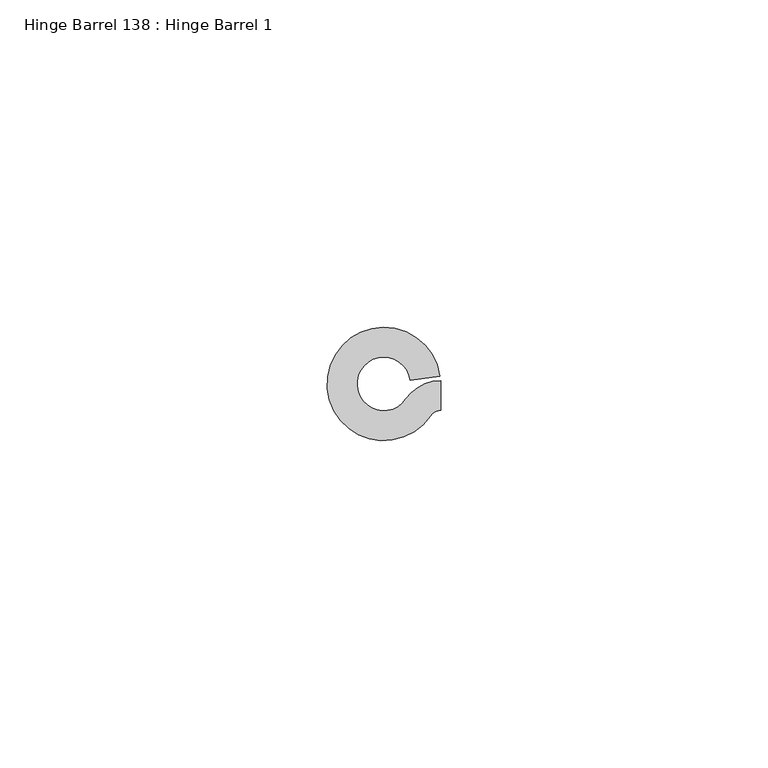
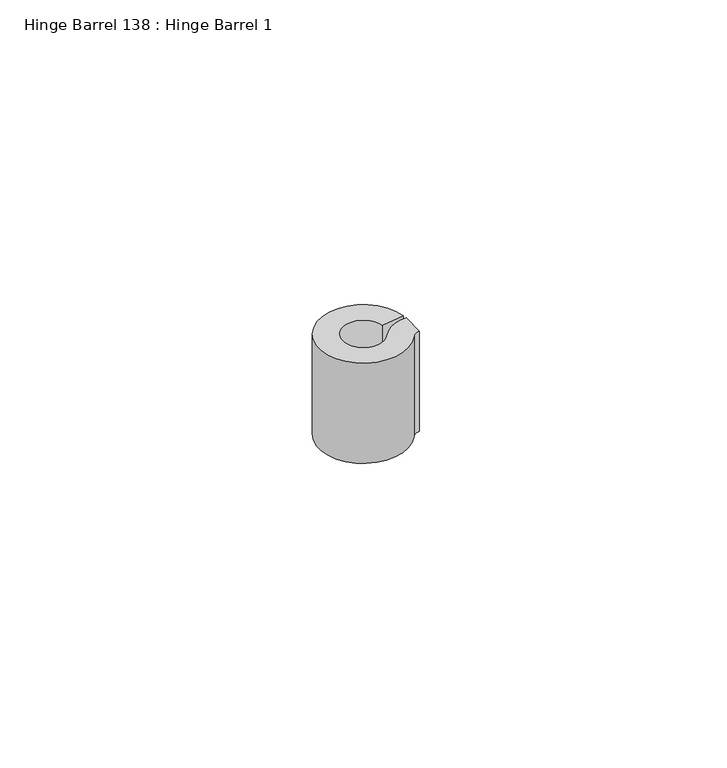
"""IFC4 building model written with IfcOpenShell, lengths in millimetres: proxy geometry, Hinge Barrel 138 : Hinge Barrel 1."""

from ifc_helpers import new_model, si_unit, point, frame, frame_2d, origin, place, context, project, spatial, polyline, circle_curve, trimmed, segment, composite_curve, outline, extrude, source, transform, mapped, element, save


def hinge_barrel_138_hinge_barrel_1_4b45ecc4(model_context):
    return source(origin(), model_context, "Body", "SweptSolid", [
        extrude(outline(composite_curve([segment(trimmed(circle_curve(frame_2d((587327.8245257, -536316.2443067)), 6.4044851), [point((587322.5194669, -536312.6563017))], [point((587327.8245257, -536309.8398216))], False, "CARTESIAN"), True, "CONTINUOUS"), segment(polyline([(587327.8245257, -536309.8398216), (587327.8245257, -536314.4038841)]), True, "CONTINUOUS"), segment(trimmed(circle_curve(frame_2d((587327.8245257, -536316.2443067)), 1.8404226), [point((587327.8245257, -536314.4038841))], [point((587326.3000393, -536315.2132409))], True, "CARTESIAN"), True, "CONTINUOUS"), segment(trimmed(circle_curve(frame_2d((587319.1320739, -536310.3652841)), 8.6534625), [point((587326.3000393, -536315.2132409))], [point((587327.7022899, -536309.1678654))], False, "CARTESIAN"), True, "CONTINUOUS"), segment(polyline([(587327.7022899, -536309.1678654), (587323.1821338, -536309.7994153)]), True, "CONTINUOUS"), segment(trimmed(circle_curve(frame_2d((587319.1320739, -536310.3652841)), 4.0894), [point((587323.1821338, -536309.7994153))], [point((587322.5194669, -536312.6563017))], True, "CARTESIAN"), True, "CONTINUOUS")], self_intersect=False)), frame((0.0, 0.0, 2063.75), z_axis=(0.0, 0.0, 1.0), x_axis=(1.0, 0.0, 0.0)), (0.0, 0.0, 1.0), 20.8359375),
    ])


if __name__ == "__main__":
    model = new_model("IFC4")
    model_context = context("Model", 3, world=origin())
    ifc_project = project(units=[si_unit("LENGTHUNIT", "METRE", prefix="MILLI")], contexts=[model_context])
    site = spatial("IfcSite", under=ifc_project)
    building = spatial("IfcBuilding", under=site)
    placement = place(None, origin())
    hinge_barrel_138_hinge_barrel_1_shape = hinge_barrel_138_hinge_barrel_1_4b45ecc4(model_context)
    element("IfcBuildingElementProxy", 1, Name="Hinge Barrel 138 : Hinge Barrel 1", ObjectType="Hinge Barrel 138 : Hinge Barrel 1", at=placement, inside=building, context=model_context, shape_type="MappedRepresentation", body=[
        mapped(hinge_barrel_138_hinge_barrel_1_shape, transform((0.0, 0.0, 0.0), x_axis=(1.0, 0.0, 0.0), y_axis=(0.0, 1.0, 0.0), z_axis=(0.0, 0.0, 1.0))),
    ])
    save(model, "model.ifc")

# Revit data of these elements
# Element 1 (IfcBuildingElementProxy, "Hinge Barrel 138 : Hinge Barrel 1")
#   Materials on its faces: "6\"X6\" WELD-ON STL BUTT HINGE"
# Materials
#   "6\"X6\" WELD-ON STL BUTT HINGE": class "Metal", colour RGB 189 187 185, transparency 0, Description = "Carbon steel", Cost = 0
